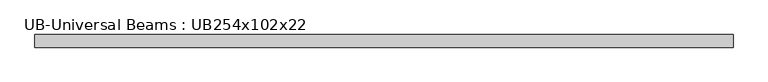
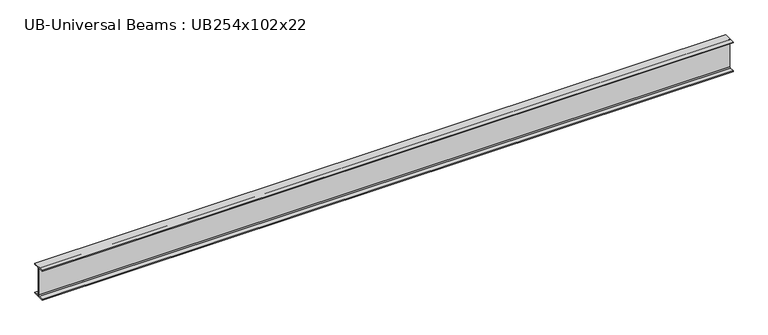
"""IFC4 building model written with IfcOpenShell, lengths in millimetres: beam geometry, UB-Universal Beams : UB254x102x22."""

from ifc_helpers import new_model, si_unit, point, frame, frame_2d, origin, place, context, project, spatial, polyline, circle_curve, trimmed, segment, composite_curve, outline, extrude, source, transform, mapped, element, save


def ub_universal_beams_ub254x102x22_5313c1c2(model_context):
    return source(origin(), model_context, "Body", "SweptSolid", [
        extrude(outline(composite_curve([segment(polyline([(50.8, -120.2), (50.8, -127.0), (-50.8, -127.0), (-50.8, -120.2), (-10.45, -120.2)]), True, "CONTINUOUS"), segment(trimmed(circle_curve(frame_2d((-10.45, -112.6)), 7.6), [point((-10.45, -120.2))], [point((-2.85, -112.6))], True, "CARTESIAN"), True, "CONTINUOUS"), segment(polyline([(-2.85, -112.6), (-2.85, 112.6)]), True, "CONTINUOUS"), segment(trimmed(circle_curve(frame_2d((-10.45, 112.6)), 7.6), [point((-2.85, 112.6))], [point((-10.45, 120.2))], True, "CARTESIAN"), True, "CONTINUOUS"), segment(polyline([(-10.45, 120.2), (-50.8, 120.2), (-50.8, 127.0), (50.8, 127.0), (50.8, 120.2), (10.45, 120.2)]), True, "CONTINUOUS"), segment(trimmed(circle_curve(frame_2d((10.45, 112.6)), 7.6), [point((10.45, 120.2))], [point((2.85, 112.6))], True, "CARTESIAN"), True, "CONTINUOUS"), segment(polyline([(2.85, 112.6), (2.85, -112.6)]), True, "CONTINUOUS"), segment(trimmed(circle_curve(frame_2d((10.45, -112.6)), 7.6), [point((2.85, -112.6))], [point((10.45, -120.2))], True, "CARTESIAN"), True, "CONTINUOUS"), segment(polyline([(10.45, -120.2), (50.8, -120.2)]), True, "CONTINUOUS")], self_intersect=False)), frame((-2834.7, 0.0, 0.0), z_axis=(1.0, 0.0, 0.0), x_axis=(0.0, 1.0, 0.0)), (0.0, 0.0, 1.0), 5597.1),
    ])


if __name__ == "__main__":
    model = new_model("IFC4")
    model_context = context("Model", 3, world=origin())
    ifc_project = project(units=[si_unit("LENGTHUNIT", "METRE", prefix="MILLI")], contexts=[model_context])
    site = spatial("IfcSite", under=ifc_project)
    building = spatial("IfcBuilding", under=site)
    placement = place(None, origin())
    ub_universal_beams_ub254x102x22_shape = ub_universal_beams_ub254x102x22_5313c1c2(model_context)
    element("IfcBeam", 1, ObjectType="UB-Universal Beams : UB254x102x22", at=placement, inside=building, context=model_context, shape_type="MappedRepresentation", body=[
        mapped(ub_universal_beams_ub254x102x22_shape, transform((0.0, 0.0, 0.0), x_axis=(1.0, 0.0, 0.0), y_axis=(0.0, 1.0, 0.0), z_axis=(0.0, 0.0, 1.0))),
    ])
    save(model, "model.ifc")

# Revit data of these elements
# Type "UB-Universal Beams : UB254x102x22"
#   Section Name Key = "UB254X102X22"
#   Width = 10.16 cm
#   Web Thickness = 0.57 cm
#   Web Fillet = 0.76 cm
#   Warping Constant = 18200.0 cm⁶
#   Torsional Moment of Inertia = 4.15 cm⁴
#   Section Area = 28.0 cm²
#   Plastic Modulus weak axis = 37.3 cm³
#   Plastic Modulus strong axis = 259.0 cm³
#   Nominal Weight = 22.00 kgf/m
#   Moment of Inertia weak axis = 119.00 cm⁴
#   Moment of Inertia strong axis = 2841.00 cm⁴
#   Height = 25.4 cm
#   Flange Thickness = 0.68 cm
#   Elastic Modulus weak axis = 23.5 cm³
#   Elastic Modulus strong axis = 224.0 cm³
#   Centroid Vertical = 12.7 cm
#   Centroid Horizontal = 5.08 cm
#   Bolt Spacing = 5.4 cm
#   Length [instance default] = 1500 mm
#   Structural Material [instance default] = Metal - Steel 43-275
#   Type Comments = ""
#   Assembly Code = ""
# Element 1 (IfcBeam, "UB-Universal Beams : UB254x102x22")
#   Materials on its faces: "Metal - Steel 43-275"
# Materials
#   "Metal - Steel 43-275": class "Metal", colour RGB 247 247 247, transparency 0, Cost = 0
